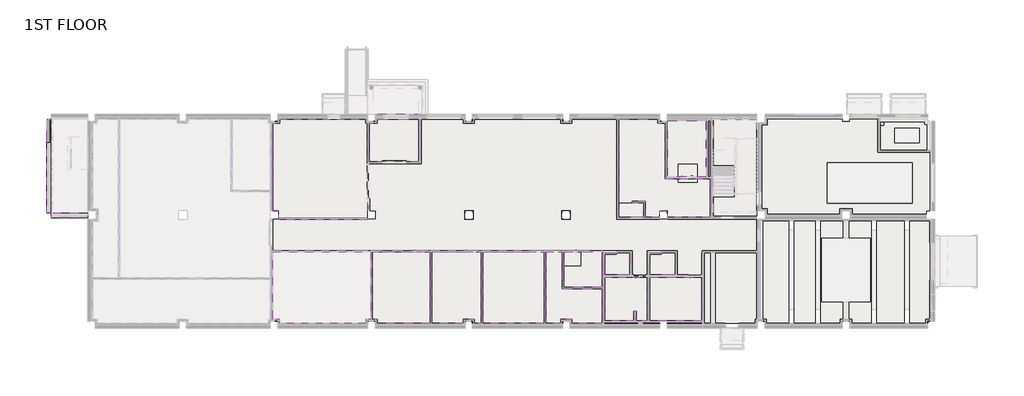
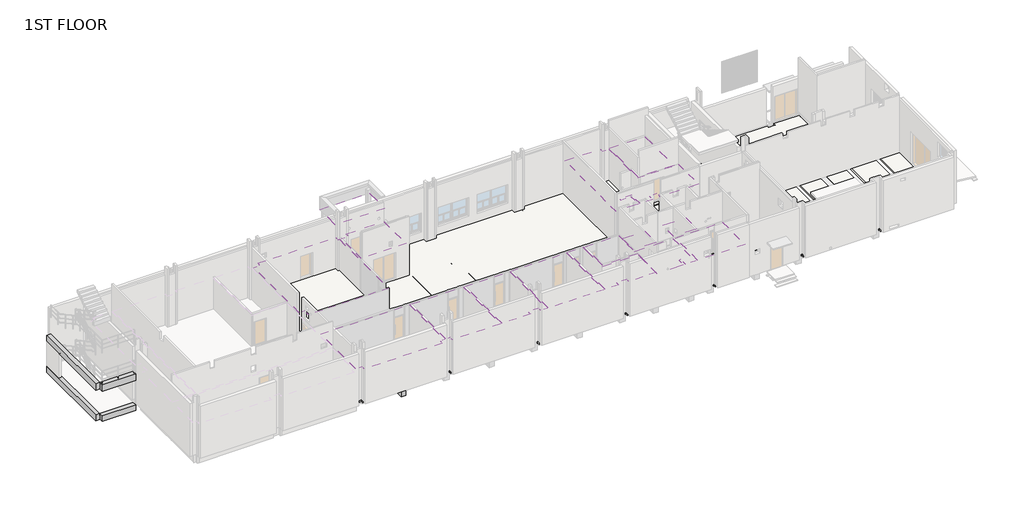
# One storey, part 8 of 15: 26 slabs, 15 coverings, 5 beams.
"""IFC4 building model written with IfcOpenShell, lengths in millimetres."""

from ifc_helpers import new_model, si_unit, frame, origin, place, context, project, spatial, polyline, outline, extrude, faceted_brep, element, save

model = new_model("IFC4")

# Units and contexts
model_context = context("Model", 3, world=origin())
ifc_project = project(units=[si_unit("LENGTHUNIT", "METRE", prefix="MILLI")], contexts=[model_context])

# Site, building, storey
site = spatial("IfcSite", under=ifc_project)
building = spatial("IfcBuilding", under=site)
storey = spatial("IfcBuildingStorey", under=building, Name="1ST FLOOR", Elevation=4800.0)

# Beams
placement = place(None, origin())
element("IfcBeam", 1, ObjectType="RC Beam_Rectangular : H_SB_AR S16_TG-UG_450x800_1B1A", at=placement, inside=storey, context=model_context, shape_type="Brep", body=[
    faceted_brep([(18775.0, -16900.0, 4800.0), (19225.0, -16900.0, 4800.0), (19225.0, -8350.0, 4800.0), (18775.0, -8350.0, 4800.0), (19225.0, -16900.0, 4650.0), (19225.0, -16900.0, 4000.0), (19225.0, -8350.0, 4000.0), (19225.0, -8350.0, 4650.0), (18775.0, -16900.0, 4000.0), (18775.0, -8350.0, 4000.0), (18775.0, -8350.0, 4650.0), (18775.0, -16900.0, 4650.0)], [[[0, 1, 2, 3]], [[2, 1, 4, 5, 6, 7]], [[5, 8, 9, 6]], [[0, 3, 10, 9, 8, 11]], [[1, 0, 11, 8, 5, 4]], [[3, 2, 7, 6, 9, 10]]]),
])
element("IfcBeam", 2, ObjectType="RC Beam_Rectangular : H_SB_AR S16_RC Beam-AG_400x530_SG1A", at=placement, inside=storey, context=model_context, shape_type="Brep", body=[
    faceted_brep([(-300.0, -8200.0, 4630.0), (-300.0, -7800.0, 4630.0), (-3300.0, -7800.0, 4630.0), (-3300.0, -8200.0, 4630.0), (-300.0, -8200.0, 4100.0), (-3300.0, -8200.0, 4100.0), (-300.0, -7800.0, 4100.0), (-3300.0, -7800.0, 4100.0), (-300.0, -7800.0, 4430.0), (-3300.0, -7800.0, 4430.0)], [[[0, 1, 2, 3]], [[4, 0, 3, 5]], [[6, 4, 5, 7]], [[1, 8, 6, 7, 9, 2]], [[1, 0, 4, 6, 8]], [[2, 9, 7, 5, 3]]]),
])
element("IfcBeam", 3, ObjectType="RC Beam_Rectangular : H_SB_AR S16_RC Beam-AG_400x600_SG2", at=placement, inside=storey, context=model_context, shape_type="Brep", body=[
    faceted_brep([(-3700.0, -7800.0, 4630.0), (-3300.0, -7800.0, 4630.0), (-3300.0, -100.0, 4630.0), (-3450.0, -100.0, 4630.0), (-3700.0, -100.0, 4630.0), (-3700.0, -2000.0, 4630.0), (-3700.0, -7800.0, 4030.0), (-3700.0, -100.0, 4030.0), (-3300.0, -7800.0, 4030.0), (-3300.0, -100.0, 4030.0), (-3300.0, -7800.0, 4430.0), (-3300.0, -100.0, 4430.0)], [[[0, 1, 2, 3, 4, 5]], [[6, 0, 5, 4, 7]], [[8, 6, 7, 9]], [[1, 10, 8, 9, 11, 2]], [[1, 0, 6, 8, 10]], [[4, 3, 2, 11, 9, 7]]]),
])
element("IfcBeam", 4, ObjectType="RC Beam_Rectangular : H_SB_AR S16_RC Beam-AG_400x600_SWG2", at=placement, inside=storey, context=model_context, shape_type="Brep", body=[
    faceted_brep([(-3700.0, -7800.0, 7590.0), (-3300.0, -7800.0, 7590.0), (-3300.0, -100.0, 7590.0), (-3450.0, -100.0, 7590.0), (-3700.0, -100.0, 7590.0), (-3700.0, -2000.0, 7590.0), (-3300.0, -7800.0, 6990.0), (-3300.0, -100.0, 6990.0), (-3700.0, -7800.0, 6990.0), (-3700.0, -2000.0, 6990.0), (-3700.0, -100.0, 6990.0), (-3450.0, -100.0, 6990.0)], [[[0, 1, 2, 3, 4, 5]], [[1, 6, 7, 2]], [[6, 8, 9, 10, 11, 7]], [[8, 0, 5, 4, 10, 9]], [[1, 0, 8, 6]], [[4, 3, 2, 7, 11, 10]]]),
])
element("IfcBeam", 5, ObjectType="RC Beam_Rectangular : H_SB_AR S16_RC Beam-AG_400x600_SG1", at=placement, inside=storey, context=model_context, shape_type="SweptSolid", body=[
    extrude(outline(polyline([(-300.0, -7800.0), (-300.0, -8200.0), (-3300.0, -8200.0), (-3300.0, -7800.0), (-300.0, -7800.0)])), frame((0.0, 0.0, 6990.0), z_axis=(0.0, 0.0, 1.0), x_axis=(1.0, 0.0, 0.0)), (0.0, 0.0, 1.0), 600.0),
])

# Coverings
element("IfcCovering", 6, ObjectType="H_CE_AR_B09_2L Gypsum Board_T Bar_9T_C4", at=placement, inside=storey, context=model_context, shape_type="SweptSolid", body=[
    extrude(outline(polyline([(22536.0, -114.0), (22536.0, -464.0), (22649.9999955, -464.0), (22649.9999955, -8250.0), (15400.0000001, -8250.0), (15400.0000001, -7650.0), (14886.0, -7650.0), (14886.0, -464.0), (15464.0, -464.0), (15464.0, -114.0), (22536.0, -114.0)])), frame((0.0, 0.0, 7830.0), z_axis=(0.0, 0.0, 1.0), x_axis=(1.0, 0.0, 0.0)), (0.0, 0.0, 1.0), 19.0),
])
element("IfcCovering", 7, ObjectType="H_CE_AR_B09_Aluminum Spandrel_M Bar_0.8T_C9", at=placement, inside=storey, context=model_context, shape_type="SweptSolid", body=[
    extrude(outline(polyline([(22836.0, -464.0), (23464.0, -464.0), (23464.0, -114.0), (26907.0, -114.0), (26907.0, -3607.0), (22836.0, -3607.0), (22836.0, -464.0)])), frame((0.0, 0.0, 7830.0), z_axis=(0.0, 0.0, 1.0), x_axis=(1.0, 0.0, 0.0)), (0.0, 0.0, 1.0), 0.8),
])
element("IfcCovering", 8, ObjectType="H_CE_AR_B09_2L Gypsum Board_T Bar_9T_C4", at=placement, inside=storey, context=model_context, shape_type="SweptSolid", body=[
    extrude(outline(polyline([(43343.0, -114.0), (46536.0, -114.0), (46536.0, -464.0), (47132.0, -464.0), (47132.0, -4993.0), (50825.0, -4993.0), (50825.0, -8164.0), (47349.9999999, -8164.0), (47349.9999999, -7650.0), (46649.9999999, -7650.0), (46649.9999999, -8164.0), (45514.0, -8164.0), (45514.0, -6836.0), (44443.0, -6836.0), (44443.0, -6964.0), (45386.0, -6964.0), (45386.0, -8164.0), (43343.0, -8164.0), (43343.0, -114.0)])), frame((0.0, 0.0, 7910.0), z_axis=(0.0, 0.0, 1.0), x_axis=(1.0, 0.0, 0.0)), (0.0, 0.0, 1.0), 19.0),
])
element("IfcCovering", 9, ObjectType="H_CE_AR_B09_SMC Ceiling_T Bar_300x300x0.8T_C6", at=placement, inside=storey, context=model_context, shape_type="SweptSolid", body=[
    extrude(outline(polyline([(50525.0, -4825.0), (47300.0, -4825.0), (47300.0, -250.0), (50525.0, -250.0), (50525.0, -4825.0)])), frame((0.0, 0.0, 7800.0), z_axis=(0.0, 0.0, 1.0), x_axis=(1.0, 0.0, 0.0)), (0.0, 0.0, 1.0), 0.8),
])
element("IfcCovering", 10, ObjectType="H_CE_AR_B09_2L Gypsum Board_T Bar_9T_C4", at=placement, inside=storey, context=model_context, shape_type="SweptSolid", body=[
    extrude(outline(polyline([(14886.0, -11007.0000083), (22936.0, -11007.0000083), (22936.0, -16536.0), (22536.0, -16536.0), (22536.0, -16886.0), (15464.0, -16886.0), (15464.0, -16536.0), (14886.0, -16536.0), (14886.0, -11007.0000083)])), frame((0.0, 0.0, 7830.0), z_axis=(0.0, 0.0, 1.0), x_axis=(1.0, 0.0, 0.0)), (0.0, 0.0, 1.0), 19.0),
])
element("IfcCovering", 11, ObjectType="H_CE_AR_B09_2L Gypsum Board_T Bar_9T_C4", at=placement, inside=storey, context=model_context, shape_type="SweptSolid", body=[
    extrude(outline(polyline([(23464.0, -16886.0), (23464.0, -16536.0), (23064.0, -16536.0), (23064.0, -11007.0), (27836.0, -11007.0), (27836.0, -16886.0), (23464.0, -16886.0)])), frame((0.0, 0.0, 7830.0), z_axis=(0.0, 0.0, 1.0), x_axis=(1.0, 0.0, 0.0)), (0.0, 0.0, 1.0), 19.0),
])
element("IfcCovering", 12, ObjectType="H_CE_AR_B09_Souns Absorbing Soft Fiber Board_T Bar_600x600x9T_C5", at=placement, inside=storey, context=model_context, shape_type="SweptSolid", body=[
    extrude(outline(polyline([(27964.0, -11007.0), (32036.0, -11007.0), (32036.0, -16886.0), (31464.0, -16886.0), (31464.0, -16536.0), (30536.0, -16536.0), (30536.0, -16886.0), (27964.0, -16886.0), (27964.0, -11007.0)])), frame((0.0, 0.0, 7830.0), z_axis=(0.0, 0.0, 1.0), x_axis=(1.0, 0.0, 0.0)), (0.0, 0.0, 1.0), 9.0),
])
element("IfcCovering", 13, ObjectType="H_CE_AR_B09_2L Gypsum Board_T Bar_9T_C4", at=placement, inside=storey, context=model_context, shape_type="SweptSolid", body=[
    extrude(outline(polyline([(37186.0, -11007.0), (37186.0, -16886.0), (32164.0, -16886.0), (32164.0, -11007.0), (37186.0, -11007.0)])), frame((0.0, 0.0, 7830.0), z_axis=(0.0, 0.0, 1.0), x_axis=(1.0, 0.0, 0.0)), (0.0, 0.0, 1.0), 19.0),
])
element("IfcCovering", 14, ObjectType="H_CE_AR_B09_Souns Absorbing Soft Fiber Board_T Bar_600x600x9T_C5", at=placement, inside=storey, context=model_context, shape_type="SweptSolid", body=[
    extrude(outline(polyline([(38686.0000001, -14064.0), (41957.0, -14064.0), (41957.0, -16886.0), (39464.0, -16886.0), (39464.0, -16536.0), (38536.0, -16536.0), (38536.0, -16886.0), (37314.0, -16886.0), (37314.0, -11007.0000083), (38686.0000001, -11007.0000083), (38686.0000001, -14064.0)])), frame((0.0, 0.0, 7830.0), z_axis=(0.0, 0.0, 1.0), x_axis=(1.0, 0.0, 0.0)), (0.0, 0.0, 1.0), 9.0),
])
element("IfcCovering", 15, ObjectType="H_CE_AR_B09_Souns Absorbing Soft Fiber Board_T Bar_600x600x9T_C5", at=placement, inside=storey, context=model_context, shape_type="SweptSolid", body=[
    extrude(outline(polyline([(41957.0, -11007.0), (41957.0, -13936.0), (38814.0000001, -13936.0), (38814.0000001, -11007.0), (41957.0, -11007.0)])), frame((0.0, 0.0, 7830.0), z_axis=(0.0, 0.0, 1.0), x_axis=(1.0, 0.0, 0.0)), (0.0, 0.0, 1.0), 9.0),
])
element("IfcCovering", 16, ObjectType="H_CE_AR_B09_2L Gypsum Board_T Bar_9T_C4", at=placement, inside=storey, context=model_context, shape_type="SweptSolid", body=[
    extrude(outline(polyline([(44245.0, -12895.0), (42155.0, -12895.0), (42155.0, -11105.0), (44245.0, -11105.0), (44245.0, -12895.0)])), frame((0.0, 0.0, 7500.0), z_axis=(0.0, 0.0, 1.0), x_axis=(1.0, 0.0, 0.0)), (0.0, 0.0, 1.0), 19.0),
])
element("IfcCovering", 17, ObjectType="H_CE_AR_B09_2L Gypsum Board_T Bar_9T_C4", at=placement, inside=storey, context=model_context, shape_type="SweptSolid", body=[
    extrude(outline(polyline([(45645.0, -13105.0), (45645.0, -16670.0), (44755.0, -16670.0), (44755.0, -15905.0), (44545.0, -15905.0), (44545.0, -16670.0), (42155.0, -16670.0), (42155.0, -13105.0), (45645.0, -13105.0)])), frame((0.0, 0.0, 7500.0), z_axis=(0.0, 0.0, 1.0), x_axis=(1.0, 0.0, 0.0)), (0.0, 0.0, 1.0), 19.0),
])
element("IfcCovering", 18, ObjectType="H_CE_AR_B09_2L Gypsum Board_T Bar_9T_C4", at=placement, inside=storey, context=model_context, shape_type="SweptSolid", body=[
    extrude(outline(polyline([(50145.0, -13105.0), (50145.0, -16670.0), (45855.0, -16670.0), (45855.0, -13105.0), (50145.0, -13105.0)])), frame((0.0, 0.0, 7500.0), z_axis=(0.0, 0.0, 1.0), x_axis=(1.0, 0.0, 0.0)), (0.0, 0.0, 1.0), 19.0),
])
element("IfcCovering", 19, ObjectType="H_CE_AR_B09_2L Gypsum Board_T Bar_9T_C4", at=placement, inside=storey, context=model_context, shape_type="SweptSolid", body=[
    extrude(outline(polyline([(47945.0, -11105.0000016), (47945.0, -12895.0), (45855.0, -12895.0), (45855.0, -11105.0000016), (47945.0, -11105.0000016)])), frame((0.0, 0.0, 7500.0), z_axis=(0.0, 0.0, 1.0), x_axis=(1.0, 0.0, 0.0)), (0.0, 0.0, 1.0), 19.0),
])
element("IfcCovering", 20, ObjectType="H_CE_AR_B09_Stainless Hairline Finish_3T", at=placement, inside=storey, context=model_context, shape_type="SweptSolid", body=[
    extrude(outline(polyline([(27247.0, 2747.0), (27247.0, 300.0), (22753.0, 300.0), (22753.0, 2747.0), (27247.0, 2747.0)]), holes=[polyline([(23150.0, 2650.0), (22850.0, 2650.0), (22850.0, 2350.0), (23150.0, 2350.0), (23150.0, 2650.0)]), polyline([(26850.0, 2650.0), (26850.0, 2350.0), (27150.0, 2350.0), (27150.0, 2650.0), (26850.0, 2650.0)])]), frame((0.0, 0.0, 8700.0), z_axis=(0.0, 0.0, 1.0), x_axis=(1.0, 0.0, 0.0)), (0.0, 0.0, 1.0), 3.0),
])

# Slabs
element("IfcSlab", 21, ObjectType="H_FL_AR_S17_RC Slab_T150_1S1", at=placement, inside=storey, context=model_context, shape_type="Brep", body=[
    faceted_brep([(18775.0, -100.0, 4650.0), (18775.0, -7850.0, 4650.0), (15400.0000001, -7850.0, 4650.0), (15400.0000001, -7650.0, 4650.0), (15100.0, -7650.0, 4650.0), (15100.0, -300.0, 4650.0), (15300.0, -300.0, 4650.0), (15300.0, -100.0, 4650.0), (18775.0, -7850.0, 4800.0), (18775.0, -100.0, 4800.0), (15300.0, -100.0, 4800.0), (15300.0, -300.0, 4800.0), (15100.0, -300.0, 4800.0), (15100.0, -7650.0, 4800.0), (15400.0000001, -7650.0, 4800.0), (15400.0000001, -7850.0, 4800.0)], [[[0, 1, 2, 3, 4, 5, 6, 7]], [[8, 9, 10, 11, 12, 13, 14, 15]], [[1, 0, 9, 8]], [[2, 1, 8, 15]], [[3, 2, 15, 14]], [[4, 3, 14, 13]], [[5, 4, 13, 12]], [[0, 7, 10, 9]], [[6, 5, 12, 11]], [[7, 6, 11, 10]]]),
    faceted_brep([(18775.0, -16900.0, 4650.0), (15300.0, -16900.0, 4650.0), (15300.0, -16700.0, 4650.0), (15100.0, -16700.0, 4650.0), (15100.0, -8350.0, 4650.0), (18775.0, -8350.0, 4650.0), (15300.0, -16900.0, 4800.0), (18775.0, -16900.0, 4800.0), (18775.0, -8350.0, 4800.0), (15400.0000001, -8350.0, 4800.0), (15100.0, -8350.0, 4800.0), (15100.0, -16700.0, 4800.0), (15300.0, -16700.0, 4800.0)], [[[0, 1, 2, 3, 4, 5]], [[6, 7, 8, 9, 10, 11, 12]], [[1, 0, 7, 6]], [[2, 1, 6, 12]], [[3, 2, 12, 11]], [[4, 3, 11, 10]], [[5, 4, 10, 9, 8]], [[0, 5, 8, 7]]]),
    faceted_brep([(22650.0000003, -7850.0, 4650.0), (19225.0, -7850.0, 4650.0), (19225.0, -100.0, 4650.0), (22700.0, -100.0, 4650.0), (22700.0, -7650.0, 4650.0), (22650.0000003, -7650.0, 4650.0), (19225.0, -7850.0, 4800.0), (22650.0000003, -7850.0, 4800.0), (22650.0000003, -7650.0, 4800.0), (22700.0, -7650.0, 4800.0), (22700.0, -300.0, 4800.0), (22700.0, -100.0, 4800.0), (19225.0, -100.0, 4800.0)], [[[0, 1, 2, 3, 4, 5]], [[6, 7, 8, 9, 10, 11, 12]], [[1, 0, 7, 6]], [[2, 1, 6, 12]], [[3, 2, 12, 11]], [[4, 3, 11, 10, 9]], [[5, 4, 9, 8]], [[0, 5, 8, 7]]]),
    faceted_brep([(19225.0, -8350.0, 4650.0), (22750.0, -8350.0, 4650.0), (22750.0, -16700.0, 4650.0), (22700.0, -16700.0, 4650.0), (22700.0, -16900.0, 4650.0), (19225.0, -16900.0, 4650.0), (22750.0, -8350.0, 4800.0), (22650.0, -8350.0, 4800.0), (19225.0, -8350.0, 4800.0), (19225.0, -16900.0, 4800.0), (22700.0, -16900.0, 4800.0), (22700.0, -16700.0, 4800.0), (22750.0, -16700.0, 4800.0)], [[[0, 1, 2, 3, 4, 5]], [[6, 7, 8, 9, 10, 11, 12]], [[1, 0, 8, 7, 6]], [[2, 1, 6, 12]], [[3, 2, 12, 11]], [[4, 3, 11, 10]], [[5, 4, 10, 9]], [[0, 5, 9, 8]]]),
    faceted_brep([(26775.0, -8350.0, 4650.0), (26775.0, -16900.0, 4650.0), (23300.0, -16900.0, 4650.0), (23300.0, -16700.0, 4650.0), (23250.0, -16700.0, 4650.0), (23250.0, -8350.0, 4650.0), (26775.0, -16900.0, 4800.0), (26775.0, -8350.0, 4800.0), (23350.0, -8350.0, 4800.0), (23250.0, -8350.0, 4800.0), (23250.0, -16700.0, 4800.0), (23300.0, -16700.0, 4800.0), (23300.0, -16900.0, 4800.0)], [[[0, 1, 2, 3, 4, 5]], [[6, 7, 8, 9, 10, 11, 12]], [[1, 0, 7, 6]], [[2, 1, 6, 12]], [[3, 2, 12, 11]], [[4, 3, 11, 10]], [[5, 4, 10, 9]], [[0, 5, 9, 8, 7]]]),
    faceted_brep([(23350.0000003, -7850.0, 4650.0), (23350.0000003, -7650.0, 4650.0), (23200.0, -7650.0, 4650.0), (23200.0, -300.0, 4650.0), (23300.0, -300.0, 4650.0), (23300.0, -100.0, 4650.0), (26775.0, -100.0, 4650.0), (26775.0, -7850.0, 4650.0), (23350.0000003, -7650.0, 4800.0), (23350.0000003, -7850.0, 4800.0), (26775.0, -7850.0, 4800.0), (26775.0, -100.0, 4800.0), (23300.0, -100.0, 4800.0), (23300.0, -300.0, 4800.0), (23200.0, -300.0, 4800.0), (23200.0, -7650.0, 4800.0)], [[[0, 1, 2, 3, 4, 5, 6, 7]], [[8, 9, 10, 11, 12, 13, 14, 15]], [[1, 0, 9, 8]], [[2, 1, 8, 15]], [[3, 2, 15, 14]], [[4, 3, 14, 13]], [[5, 4, 13, 12]], [[6, 5, 12, 11]], [[7, 6, 11, 10]], [[0, 7, 10, 9]]]),
    faceted_brep([(30700.0, -100.0, 4650.0), (30700.0, -300.0, 4650.0), (30750.0, -300.0, 4650.0), (30750.0, -7650.0, 4650.0), (30650.0000002, -7650.0, 4650.0), (30650.0000002, -7850.0, 4650.0), (27225.0, -7850.0, 4650.0), (27225.0, -100.0, 4650.0), (30700.0, -300.0, 4800.0), (30700.0, -100.0, 4800.0), (27225.0, -100.0, 4800.0), (27225.0, -7850.0, 4800.0), (30650.0000002, -7850.0, 4800.0), (30650.0000002, -7650.0, 4800.0), (30750.0, -7650.0, 4800.0), (30750.0, -300.0, 4800.0)], [[[0, 1, 2, 3, 4, 5, 6, 7]], [[8, 9, 10, 11, 12, 13, 14, 15]], [[1, 0, 9, 8]], [[2, 1, 8, 15]], [[3, 2, 15, 14]], [[4, 3, 14, 13]], [[5, 4, 13, 12]], [[6, 5, 12, 11]], [[7, 6, 11, 10]], [[0, 7, 10, 9]]]),
    faceted_brep([(30700.0, -16900.0, 4650.0), (27225.0, -16900.0, 4650.0), (27225.0, -8350.0, 4650.0), (30750.0, -8350.0, 4650.0), (30750.0, -16700.0, 4650.0), (30700.0, -16700.0, 4650.0), (27225.0, -16900.0, 4800.0), (30700.0, -16900.0, 4800.0), (30700.0, -16700.0, 4800.0), (30750.0, -16700.0, 4800.0), (30750.0, -8350.0, 4800.0), (30650.0, -8350.0, 4800.0), (27225.0, -8350.0, 4800.0)], [[[0, 1, 2, 3, 4, 5]], [[6, 7, 8, 9, 10, 11, 12]], [[1, 0, 7, 6]], [[2, 1, 6, 12]], [[3, 2, 12, 11, 10]], [[4, 3, 10, 9]], [[5, 4, 9, 8]], [[0, 5, 8, 7]]]),
    faceted_brep([(31300.0, -16900.0, 4650.0), (31300.0, -16700.0, 4650.0), (31250.0, -16700.0, 4650.0), (31250.0, -8350.0, 4650.0), (34775.0, -8350.0, 4650.0), (34775.0, -16900.0, 4650.0), (31300.0, -16700.0, 4800.0), (31300.0, -16900.0, 4800.0), (34775.0, -16900.0, 4800.0), (34775.0, -8350.0, 4800.0), (31350.0, -8350.0, 4800.0), (31250.0, -8350.0, 4800.0), (31250.0, -16700.0, 4800.0)], [[[0, 1, 2, 3, 4, 5]], [[6, 7, 8, 9, 10, 11, 12]], [[1, 0, 7, 6]], [[2, 1, 6, 12]], [[3, 2, 12, 11]], [[4, 3, 11, 10, 9]], [[5, 4, 9, 8]], [[0, 5, 8, 7]]]),
    faceted_brep([(31300.0, -100.0, 4650.0), (34775.0, -100.0, 4650.0), (34775.0, -7850.0, 4650.0), (31349.9999998, -7850.0, 4650.0), (31349.9999998, -7650.0, 4650.0), (31250.0, -7650.0, 4650.0), (31250.0, -300.0, 4650.0), (31300.0, -300.0, 4650.0), (34775.0, -100.0, 4800.0), (31300.0, -100.0, 4800.0), (31300.0, -300.0, 4800.0), (31250.0, -300.0, 4800.0), (31250.0, -7650.0, 4800.0), (31349.9999998, -7650.0, 4800.0), (31349.9999998, -7850.0, 4800.0), (34775.0, -7850.0, 4800.0)], [[[0, 1, 2, 3, 4, 5, 6, 7]], [[8, 9, 10, 11, 12, 13, 14, 15]], [[1, 0, 9, 8]], [[2, 1, 8, 15]], [[3, 2, 15, 14]], [[4, 3, 14, 13]], [[5, 4, 13, 12]], [[6, 5, 12, 11]], [[7, 6, 11, 10]], [[0, 7, 10, 9]]]),
    faceted_brep([(38700.0, -16900.0, 4650.0), (35225.0, -16900.0, 4650.0), (35225.0, -8350.0, 4650.0), (38750.0, -8350.0, 4650.0), (38750.0, -16700.0, 4650.0), (38700.0, -16700.0, 4650.0), (35225.0, -16900.0, 4800.0), (38700.0, -16900.0, 4800.0), (38700.0, -16700.0, 4800.0), (38750.0, -16700.0, 4800.0), (38750.0, -8350.0, 4800.0), (38650.0, -8350.0, 4800.0), (35225.0, -8350.0, 4800.0)], [[[0, 1, 2, 3, 4, 5]], [[6, 7, 8, 9, 10, 11, 12]], [[1, 0, 7, 6]], [[2, 1, 6, 12]], [[3, 2, 12, 11, 10]], [[4, 3, 10, 9]], [[5, 4, 9, 8]], [[0, 5, 8, 7]]]),
    faceted_brep([(38700.0, -100.0, 4650.0), (38700.0, -300.0, 4650.0), (38750.0, -300.0, 4650.0), (38750.0, -7650.0, 4650.0), (38650.0000002, -7650.0, 4650.0), (38650.0000002, -7850.0, 4650.0), (35225.0, -7850.0, 4650.0), (35225.0, -100.0, 4650.0), (38700.0, -300.0, 4800.0), (38700.0, -100.0, 4800.0), (35225.0, -100.0, 4800.0), (35225.0, -7850.0, 4800.0), (38650.0000002, -7850.0, 4800.0), (38650.0000002, -7650.0, 4800.0), (38750.0, -7650.0, 4800.0), (38750.0, -300.0, 4800.0)], [[[0, 1, 2, 3, 4, 5, 6, 7]], [[8, 9, 10, 11, 12, 13, 14, 15]], [[1, 0, 9, 8]], [[2, 1, 8, 15]], [[3, 2, 15, 14]], [[4, 3, 14, 13]], [[5, 4, 13, 12]], [[6, 5, 12, 11]], [[7, 6, 11, 10]], [[0, 7, 10, 9]]]),
    faceted_brep([(39300.0, -16900.0, 4650.0), (39300.0, -16700.0, 4650.0), (39250.0, -16700.0, 4650.0), (39250.0, -8350.0, 4650.0), (41675.0, -8350.0, 4650.0), (41675.0, -16900.0, 4650.0), (39300.0, -16700.0, 4800.0), (39300.0, -16900.0, 4800.0), (41675.0, -16900.0, 4800.0), (41675.0, -8350.0, 4800.0), (39350.0, -8350.0, 4800.0), (39250.0, -8350.0, 4800.0), (39250.0, -16700.0, 4800.0)], [[[0, 1, 2, 3, 4, 5]], [[6, 7, 8, 9, 10, 11, 12]], [[1, 0, 7, 6]], [[2, 1, 6, 12]], [[3, 2, 12, 11]], [[4, 3, 11, 10, 9]], [[5, 4, 9, 8]], [[0, 5, 8, 7]]]),
    faceted_brep([(39300.0, -100.0, 4650.0), (41675.0, -100.0, 4650.0), (41675.0, -7850.0, 4650.0), (39349.9999998, -7850.0, 4650.0), (39349.9999998, -7650.0, 4650.0), (39250.0, -7650.0, 4650.0), (39250.0, -300.0, 4650.0), (39300.0, -300.0, 4650.0), (41675.0, -100.0, 4800.0), (39300.0, -100.0, 4800.0), (39300.0, -300.0, 4800.0), (39250.0, -300.0, 4800.0), (39250.0, -7650.0, 4800.0), (39349.9999998, -7650.0, 4800.0), (39349.9999998, -7850.0, 4800.0), (41675.0, -7850.0, 4800.0)], [[[0, 1, 2, 3, 4, 5, 6, 7]], [[8, 9, 10, 11, 12, 13, 14, 15]], [[1, 0, 9, 8]], [[2, 1, 8, 15]], [[3, 2, 15, 14]], [[4, 3, 14, 13]], [[5, 4, 13, 12]], [[6, 5, 12, 11]], [[7, 6, 11, 10]], [[0, 7, 10, 9]]]),
    faceted_brep([(42125.0, -100.0, 4650.0), (44875.0, -100.0, 4650.0), (44875.0, -7850.0, 4650.0), (42125.0, -7850.0, 4650.0), (44875.0, -100.0, 4800.0), (42125.0, -100.0, 4800.0), (42125.0, -7850.0, 4800.0), (44875.0, -7850.0, 4800.0)], [[[0, 1, 2, 3]], [[4, 5, 6, 7]], [[1, 0, 5, 4]], [[2, 1, 4, 7]], [[3, 2, 7, 6]], [[0, 3, 6, 5]]]),
    faceted_brep([(46649.9999999, -7850.0, 4650.0), (45325.0, -7850.0, 4650.0), (45325.0, -100.0, 4650.0), (46700.0, -100.0, 4650.0), (46700.0, -300.0, 4650.0), (46800.0, -300.0, 4650.0), (46800.0, -7650.0, 4650.0), (46649.9999999, -7650.0, 4650.0), (45325.0, -7850.0, 4800.0), (46649.9999999, -7850.0, 4800.0), (46649.9999999, -7650.0, 4800.0), (46800.0, -7650.0, 4800.0), (46800.0, -300.0, 4800.0), (46700.0, -300.0, 4800.0), (46700.0, -100.0, 4800.0), (45325.0, -100.0, 4800.0)], [[[0, 1, 2, 3, 4, 5, 6, 7]], [[8, 9, 10, 11, 12, 13, 14, 15]], [[1, 0, 9, 8]], [[2, 1, 8, 15]], [[3, 2, 15, 14]], [[4, 3, 14, 13]], [[5, 4, 13, 12]], [[6, 5, 12, 11]], [[7, 6, 11, 10]], [[0, 7, 10, 9]]]),
    faceted_brep([(50825.0, -4825.0, 4650.0), (50825.0, -7850.0, 4650.0), (47349.9999999, -7850.0, 4650.0), (47300.0, -7850.0, 4650.0), (47300.0, -7650.0, 4650.0), (47300.0, -4825.0, 4650.0), (50825.0, -7850.0, 4800.0), (50825.0, -4825.0, 4800.0), (47300.0, -4825.0, 4800.0), (47300.0, -7650.0, 4800.0), (47300.0, -7850.0, 4800.0), (47349.9999999, -7850.0, 4800.0), (50825.0, -4825.0, 4700.0), (47300.0, -4825.0, 4700.0)], [[[0, 1, 2, 3, 4, 5]], [[6, 7, 8, 9, 10, 11]], [[1, 0, 12, 7, 6]], [[3, 2, 1, 6, 11, 10]], [[5, 4, 3, 10, 9, 8, 13]], [[0, 5, 13, 8, 7, 12]]]),
    faceted_brep([(54700.0, -8350.0, 4650.0), (54700.0, -16900.0, 4650.0), (51275.0, -16900.0, 4650.0), (51275.0, -8350.0, 4650.0), (54700.0, -16900.0, 4800.0), (54700.0, -16700.0, 4800.0), (54700.0, -8350.0, 4800.0), (51275.0, -8350.0, 4800.0), (51275.0, -16900.0, 4800.0)], [[[0, 1, 2, 3]], [[4, 5, 6, 7, 8]], [[1, 0, 6, 5, 4]], [[2, 1, 4, 8]], [[3, 2, 8, 7]], [[0, 3, 7, 6]]]),
    faceted_brep([(57275.0, -8350.0, 4650.0), (57275.0, -16900.0, 4650.0), (55300.0, -16900.0, 4650.0), (55300.0, -16700.0, 4650.0), (55200.0, -16700.0, 4650.0), (55200.0, -8350.0, 4650.0), (57275.0, -16900.0, 4800.0), (57275.0, -8350.0, 4800.0), (55200.0, -8350.0, 4800.0), (55200.0, -16700.0, 4800.0), (55300.0, -16700.0, 4800.0), (55300.0, -16900.0, 4800.0)], [[[0, 1, 2, 3, 4, 5]], [[6, 7, 8, 9, 10, 11]], [[1, 0, 7, 6]], [[2, 1, 6, 11]], [[3, 2, 11, 10]], [[4, 3, 10, 9]], [[5, 4, 9, 8]], [[0, 5, 8, 7]]]),
    faceted_brep([(59475.0, -8350.0, 4650.0), (59475.0, -16900.0, 4650.0), (57725.0, -16900.0, 4650.0), (57725.0, -8350.0, 4650.0), (59475.0, -16900.0, 4800.0), (59475.0, -8350.0, 4800.0), (57725.0, -8350.0, 4800.0), (57725.0, -16900.0, 4800.0)], [[[0, 1, 2, 3]], [[4, 5, 6, 7]], [[1, 0, 5, 4]], [[2, 1, 4, 7]], [[3, 2, 7, 6]], [[0, 3, 6, 5]]]),
    faceted_brep([(61750.0, -8350.0, 4650.0), (61750.0, -16700.0, 4650.0), (61700.0, -16700.0, 4650.0), (61700.0, -16900.0, 4650.0), (59925.0, -16900.0, 4650.0), (59925.0, -8350.0, 4650.0), (61750.0, -16700.0, 4800.0), (61750.0, -8350.0, 4800.0), (59925.0, -8350.0, 4800.0), (59925.0, -16900.0, 4800.0), (61700.0, -16900.0, 4800.0), (61700.0, -16700.0, 4800.0)], [[[0, 1, 2, 3, 4, 5]], [[6, 7, 8, 9, 10, 11]], [[1, 0, 7, 6]], [[2, 1, 6, 11]], [[3, 2, 11, 10]], [[4, 3, 10, 9]], [[5, 4, 9, 8]], [[0, 5, 8, 7]]]),
    faceted_brep([(62250.0, -8350.0, 4650.0), (64075.0, -8350.0, 4650.0), (64075.0, -16900.0, 4650.0), (62300.0, -16900.0, 4650.0), (62300.0, -16700.0, 4650.0), (62250.0, -16700.0, 4650.0), (64075.0, -8350.0, 4800.0), (62250.0, -8350.0, 4800.0), (62250.0, -16700.0, 4800.0), (62300.0, -16700.0, 4800.0), (62300.0, -16900.0, 4800.0), (64075.0, -16900.0, 4800.0)], [[[0, 1, 2, 3, 4, 5]], [[6, 7, 8, 9, 10, 11]], [[1, 0, 7, 6]], [[2, 1, 6, 11]], [[3, 2, 11, 10]], [[4, 3, 10, 9]], [[5, 4, 9, 8]], [[0, 5, 8, 7]]]),
    faceted_brep([(66775.0, -8350.0, 4650.0), (66775.0, -16900.0, 4650.0), (64525.0, -16900.0, 4650.0), (64525.0, -8350.0, 4650.0), (66775.0, -16900.0, 4800.0), (66775.0, -8350.0, 4800.0), (64525.0, -8350.0, 4800.0), (64525.0, -16900.0, 4800.0)], [[[0, 1, 2, 3]], [[4, 5, 6, 7]], [[1, 0, 5, 4]], [[2, 1, 4, 7]], [[3, 2, 7, 6]], [[0, 3, 6, 5]]]),
    faceted_brep([(68700.0, -16900.0, 4650.0), (67225.0, -16900.0, 4650.0), (67225.0, -8350.0, 4650.0), (68900.0, -8350.0, 4650.0), (68900.0, -16700.0, 4650.0), (68700.0, -16700.0, 4650.0), (67225.0, -16900.0, 4800.0), (68700.0, -16900.0, 4800.0), (68700.0, -16700.0, 4800.0), (68900.0, -16700.0, 4800.0), (68900.0, -8350.0, 4800.0), (67225.0, -8350.0, 4800.0)], [[[0, 1, 2, 3, 4, 5]], [[6, 7, 8, 9, 10, 11]], [[1, 0, 7, 6]], [[2, 1, 6, 11]], [[3, 2, 11, 10]], [[4, 3, 10, 9]], [[5, 4, 9, 8]], [[0, 5, 8, 7]]]),
    faceted_brep([(47250.0, -11075.0, 4650.0), (47250.0, -10675.0, 4650.0), (47250.0, -8350.0, 4650.0), (50825.0, -8350.0, 4650.0), (50825.0, -16900.0, 4650.0), (50575.0, -16900.0, 4650.0), (50175.0, -16900.0, 4650.0), (50175.0, -13075.0, 4650.0), (47975.0, -13075.0, 4650.0), (47975.0, -11075.0, 4650.0), (47250.0, -8350.0, 4800.0), (47250.0, -11075.0, 4800.0), (47975.0, -11075.0, 4800.0), (47975.0, -13075.0, 4800.0), (50175.0, -13075.0, 4800.0), (50175.0, -16900.0, 4800.0), (50825.0, -16900.0, 4800.0), (50825.0, -8350.0, 4800.0), (47350.0, -8350.0, 4800.0), (47250.0, -11075.0, 4700.0), (50175.0, -16900.0, 4700.0), (50175.0, -13075.0, 4700.0), (47975.0, -13075.0, 4700.0), (47975.0, -11075.0, 4700.0)], [[[0, 1, 2, 3, 4, 5, 6, 7, 8, 9]], [[10, 11, 12, 13, 14, 15, 16, 17, 18]], [[2, 1, 0, 19, 11, 10]], [[3, 2, 10, 18, 17]], [[4, 3, 17, 16]], [[6, 5, 4, 16, 15, 20]], [[7, 6, 20, 15, 14, 21]], [[8, 7, 21, 14, 13, 22]], [[9, 8, 22, 13, 12, 23]], [[0, 9, 23, 12, 11, 19]]]),
    faceted_brep([(46750.0, -8350.0, 4650.0), (46750.0, -10675.0, 4650.0), (46750.0, -11075.0, 4650.0), (45825.0, -11075.0, 4650.0), (45825.0, -13075.0, 4650.0), (45325.0, -13075.0, 4650.0), (45325.0, -12675.0, 4650.0), (45325.0, -8350.0, 4650.0), (46750.0, -11075.0, 4800.0), (46750.0, -8350.0, 4800.0), (46650.0, -8350.0, 4800.0), (45325.0, -8350.0, 4800.0), (45325.0, -13075.0, 4800.0), (45825.0, -13075.0, 4800.0), (45825.0, -11075.0, 4800.0), (46750.0, -11075.0, 4700.0), (45825.0, -11075.0, 4700.0), (45825.0, -13075.0, 4700.0), (45325.0, -13075.0, 4700.0)], [[[0, 1, 2, 3, 4, 5, 6, 7]], [[8, 9, 10, 11, 12, 13, 14]], [[2, 1, 0, 9, 8, 15]], [[3, 2, 15, 8, 14, 16]], [[4, 3, 16, 14, 13, 17]], [[5, 4, 17, 13, 12, 18]], [[7, 6, 5, 18, 12, 11]], [[0, 7, 11, 10, 9]]]),
    faceted_brep([(44875.0, -8350.0, 4650.0), (44875.0, -12675.0, 4650.0), (44875.0, -13075.0, 4650.0), (44275.0, -13075.0, 4650.0), (44275.0, -11075.0, 4650.0), (42125.0, -11075.0, 4650.0), (42125.0, -10675.0, 4650.0), (42125.0, -8350.0, 4650.0), (44875.0, -13075.0, 4800.0), (44875.0, -8350.0, 4800.0), (42125.0, -8350.0, 4800.0), (42125.0, -11075.0, 4800.0), (44275.0, -11075.0, 4800.0), (44275.0, -13075.0, 4800.0), (44875.0, -13075.0, 4700.0), (44275.0, -13075.0, 4700.0), (44275.0, -11075.0, 4700.0), (42125.0, -11075.0, 4700.0)], [[[0, 1, 2, 3, 4, 5, 6, 7]], [[8, 9, 10, 11, 12, 13]], [[2, 1, 0, 9, 8, 14]], [[3, 2, 14, 8, 13, 15]], [[4, 3, 15, 13, 12, 16]], [[5, 4, 16, 12, 11, 17]], [[7, 6, 5, 17, 11, 10]], [[0, 7, 10, 9]]]),
])
element("IfcSlab", 22, ObjectType="H_FL_AR_S17_RC Slab_T150_1S1", at=placement, inside=storey, context=model_context, shape_type="Brep", body=[
    faceted_brep([(50825.0, -100.0, 4550.0), (50825.0, -4825.0, 4550.0), (47300.0, -4825.0, 4550.0), (47300.0, -100.0, 4550.0), (50825.0, -100.0, 4700.0), (47300.0, -100.0, 4700.0), (47300.0, -4825.0, 4700.0), (50825.0, -4825.0, 4700.0), (50825.0, -4825.0, 4650.0), (47300.0, -4825.0, 4650.0)], [[[0, 1, 2, 3]], [[4, 5, 6, 7]], [[1, 0, 4, 7, 8]], [[2, 1, 8, 7, 6, 9]], [[3, 2, 9, 6, 5]], [[0, 3, 5, 4]]]),
])
element("IfcSlab", 23, ObjectType="H_FL_AR_S17_RC Slab_T150_GS1", at=placement, inside=storey, context=model_context, shape_type="Brep", body=[
    faceted_brep([(62312.0, -112.0, 4650.0), (64707.0, -112.0, 4650.0), (64707.0, -1062.0, 4650.0), (64707.0, -2743.0, 4650.0), (68888.0, -2743.0, 4650.0), (68888.0, -3093.0, 4650.0), (68888.0, -7638.0, 4650.0), (68588.0, -7638.0, 4650.0), (68588.0, -7938.0, 4650.0), (62362.0, -7938.0, 4650.0), (62362.0, -7638.0, 4650.0), (61638.0, -7638.0, 4650.0), (61638.0, -7938.0, 4650.0), (55362.0, -7938.0, 4650.0), (55362.0, -7638.0, 4650.0), (55062.0, -7638.0, 4650.0), (55062.0, -412.0, 4650.0), (55362.0, -412.0, 4650.0), (55362.0, -112.0, 4650.0), (61688.0, -112.0, 4650.0), (61688.0, -312.0, 4650.0), (62312.0, -312.0, 4650.0), (67450.0, -3700.0, 4650.0), (60450.0, -3700.0, 4650.0), (60450.0, -7000.0, 4650.0), (67450.0, -7000.0, 4650.0), (64707.0, -112.0, 4800.0), (62312.0, -112.0, 4800.0), (62312.0, -312.0, 4800.0), (61688.0, -312.0, 4800.0), (61688.0, -112.0, 4800.0), (55362.0, -112.0, 4800.0), (55362.0, -412.0, 4800.0), (55062.0, -412.0, 4800.0), (55062.0, -7638.0, 4800.0), (55362.0, -7638.0, 4800.0), (55362.0, -7938.0, 4800.0), (61638.0, -7938.0, 4800.0), (61638.0, -7638.0, 4800.0), (62362.0, -7638.0, 4800.0), (62362.0, -7938.0, 4800.0), (68588.0, -7938.0, 4800.0), (68588.0, -7638.0, 4800.0), (68888.0, -7638.0, 4800.0), (68888.0, -2743.0, 4800.0), (64707.0, -2743.0, 4800.0), (60450.0, -3700.0, 4800.0), (67450.0, -3700.0, 4800.0), (67450.0, -7000.0, 4800.0), (60450.0, -7000.0, 4800.0)], [[[0, 1, 2, 3, 4, 5, 6, 7, 8, 9, 10, 11, 12, 13, 14, 15, 16, 17, 18, 19, 20, 21], [22, 23, 24, 25]], [[26, 27, 28, 29, 30, 31, 32, 33, 34, 35, 36, 37, 38, 39, 40, 41, 42, 43, 44, 45], [46, 47, 48, 49]], [[1, 0, 27, 26]], [[6, 5, 4, 44, 43]], [[7, 6, 43, 42]], [[8, 7, 42, 41]], [[9, 8, 41, 40]], [[10, 9, 40, 39]], [[11, 10, 39, 38]], [[12, 11, 38, 37]], [[13, 12, 37, 36]], [[14, 13, 36, 35]], [[15, 14, 35, 34]], [[16, 15, 34, 33]], [[17, 16, 33, 32]], [[18, 17, 32, 31]], [[19, 18, 31, 30]], [[20, 19, 30, 29]], [[21, 20, 29, 28]], [[0, 21, 28, 27]], [[23, 22, 47, 46]], [[24, 23, 46, 49]], [[25, 24, 49, 48]], [[22, 25, 48, 47]], [[3, 2, 1, 26, 45]], [[4, 3, 45, 44]]]),
])
element("IfcSlab", 24, ObjectType="H_FL_AR_S17_RC Slab_T150_1S1", at=placement, inside=storey, context=model_context, shape_type="Brep", body=[
    faceted_brep([(47975.0, -11075.0, 4550.0), (47975.0, -13075.0, 4550.0), (50175.0, -13075.0, 4550.0), (50175.0, -16900.0, 4550.0), (47300.0, -16900.0, 4550.0), (47300.0, -16700.0, 4550.0), (47250.0, -16700.0, 4550.0), (47250.0, -11075.0, 4550.0), (47975.0, -11075.0, 4700.0), (47250.0, -11075.0, 4700.0), (47250.0, -16700.0, 4700.0), (47300.0, -16700.0, 4700.0), (47300.0, -16900.0, 4700.0), (50175.0, -16900.0, 4700.0), (50175.0, -13075.0, 4700.0), (47975.0, -13075.0, 4700.0), (47975.0, -11075.0, 4650.0), (47975.0, -13075.0, 4650.0), (50175.0, -13075.0, 4650.0), (50175.0, -16900.0, 4650.0), (47250.0, -11075.0, 4650.0)], [[[0, 1, 2, 3, 4, 5, 6, 7]], [[8, 9, 10, 11, 12, 13, 14, 15]], [[1, 0, 16, 8, 15, 17]], [[2, 1, 17, 15, 14, 18]], [[3, 2, 18, 14, 13, 19]], [[4, 3, 19, 13, 12]], [[5, 4, 12, 11]], [[6, 5, 11, 10]], [[7, 6, 10, 9, 20]], [[0, 7, 20, 9, 8, 16]]]),
    faceted_brep([(45325.0, -13075.0, 4550.0), (45825.0, -13075.0, 4550.0), (45825.0, -11075.0, 4550.0), (46750.0, -11075.0, 4550.0), (46750.0, -16700.0, 4550.0), (46700.0, -16700.0, 4550.0), (46700.0, -16900.0, 4550.0), (45325.0, -16900.0, 4550.0), (45325.0, -13075.0, 4700.0), (45325.0, -16900.0, 4700.0), (46700.0, -16900.0, 4700.0), (46700.0, -16700.0, 4700.0), (46750.0, -16700.0, 4700.0), (46750.0, -11075.0, 4700.0), (45825.0, -11075.0, 4700.0), (45825.0, -13075.0, 4700.0), (45325.0, -13075.0, 4650.0), (45825.0, -13075.0, 4650.0), (45825.0, -11075.0, 4650.0), (46750.0, -11075.0, 4650.0)], [[[0, 1, 2, 3, 4, 5, 6, 7]], [[8, 9, 10, 11, 12, 13, 14, 15]], [[1, 0, 16, 8, 15, 17]], [[2, 1, 17, 15, 14, 18]], [[3, 2, 18, 14, 13, 19]], [[4, 3, 19, 13, 12]], [[5, 4, 12, 11]], [[6, 5, 11, 10]], [[7, 6, 10, 9]], [[0, 7, 9, 8, 16]]]),
    faceted_brep([(44275.0, -11075.0, 4550.0), (44275.0, -13075.0, 4550.0), (44875.0, -13075.0, 4550.0), (44875.0, -16900.0, 4550.0), (42125.0, -16900.0, 4550.0), (42125.0, -11075.0, 4550.0), (44275.0, -11075.0, 4700.0), (42125.0, -11075.0, 4700.0), (42125.0, -16900.0, 4700.0), (44875.0, -16900.0, 4700.0), (44875.0, -13075.0, 4700.0), (44275.0, -13075.0, 4700.0), (44275.0, -11075.0, 4650.0), (44275.0, -13075.0, 4650.0), (44875.0, -13075.0, 4650.0), (42125.0, -11075.0, 4650.0)], [[[0, 1, 2, 3, 4, 5]], [[6, 7, 8, 9, 10, 11]], [[1, 0, 12, 6, 11, 13]], [[2, 1, 13, 11, 10, 14]], [[3, 2, 14, 10, 9]], [[4, 3, 9, 8]], [[5, 4, 8, 7, 15]], [[0, 5, 15, 7, 6, 12]]]),
])
element("IfcSlab", 25, ObjectType="H_FL_AR_S17_RC Slab_T200_SS1", at=placement, inside=storey, context=model_context, shape_type="SweptSolid", body=[
    extrude(outline(polyline([(54650.0, -100.0), (54650.0, -7950.0), (51225.0, -7950.0), (51225.0, -100.0), (54650.0, -100.0)])), frame((0.0, 0.0, 4600.0), z_axis=(0.0, 0.0, 1.0), x_axis=(1.0, 0.0, 0.0)), (0.0, 0.0, 1.0), 200.0),
])
element("IfcSlab", 26, ObjectType="H_FL_AR_S17_RC Slab_T150_GS1", at=placement, inside=storey, context=model_context, shape_type="Brep", body=[
    faceted_brep([(68688.0, -112.0, 4650.0), (68688.0, -312.0, 4650.0), (68888.0, -312.0, 4650.0), (68888.0, -2393.0, 4650.0), (68888.0, -2743.0, 4650.0), (64707.0, -2743.0, 4650.0), (64707.0, -1062.0, 4650.0), (64707.0, -112.0, 4650.0), (65257.0, -112.0, 4650.0), (65557.0, -112.0, 4650.0), (64807.0, -612.0, 4650.0), (65107.0, -612.0, 4650.0), (65107.0, -312.0, 4650.0), (64807.0, -312.0, 4650.0), (68688.0, -112.0, 4800.0), (68488.0, -112.0, 4800.0), (64707.0, -112.0, 4800.0), (64707.0, -2743.0, 4800.0), (68888.0, -2743.0, 4800.0), (68888.0, -312.0, 4800.0), (68688.0, -312.0, 4800.0), (64807.0, -612.0, 4800.0), (64807.0, -312.0, 4800.0), (65107.0, -312.0, 4800.0), (65107.0, -612.0, 4800.0)], [[[0, 1, 2, 3, 4, 5, 6, 7, 8, 9], [10, 11, 12, 13]], [[14, 15, 16, 17, 18, 19, 20], [21, 22, 23, 24]], [[1, 0, 14, 20]], [[2, 1, 20, 19]], [[4, 3, 2, 19, 18]], [[5, 4, 18, 17]], [[7, 6, 5, 17, 16]], [[0, 9, 8, 7, 16, 15, 14]], [[11, 10, 21, 24]], [[12, 11, 24, 23]], [[13, 12, 23, 22]], [[10, 13, 22, 21]]]),
])
element("IfcSlab", 27, ObjectType="H_FL_AR_B07_Wood Tile_600x600xT3_F8", at=placement, inside=storey, context=model_context, shape_type="SweptSolid", body=[
    extrude(outline(polyline([(15464.0, -464.0), (15464.0, -114.0), (22536.0, -114.0), (22536.0, -464.0), (22650.0, -464.0), (22650.0, -3793.0), (22749.9999955, -3793.0), (22749.9999955, -7650.0), (22650.0, -7650.0), (22650.0, -8350.0), (15400.0000001, -8350.0), (15400.0000001, -7650.0), (14886.0, -7650.0), (14886.0, -464.0), (15464.0, -464.0)])), frame((0.0, 0.0, 4800.0), z_axis=(0.0, 0.0, 1.0), x_axis=(1.0, 0.0, 0.0)), (0.0, 0.0, 1.0), 30.0),
])
element("IfcSlab", 28, ObjectType="H_FL_AR_B07_Deco Tile_600x600xT3", at=placement, inside=storey, context=model_context, shape_type="SweptSolid", body=[
    extrude(outline(polyline([(23350.0000003, -8350.0), (23350.0000003, -7650.0), (22749.9999955, -7650.0), (22749.9999955, -3793.0), (27093.0, -3793.0), (27093.0, -114.0), (30536.0, -114.0), (30536.0, -464.0), (31464.0, -464.0), (31464.0, -114.0), (38536.0, -114.0), (38536.0, -464.0), (39464.0, -464.0), (39464.0, -114.0), (43157.0, -114.0), (43157.0, -8350.0), (54650.0, -8350.0), (54650.0, -10907.0), (50157.0, -10907.0), (50157.0, -12907.0), (48143.0, -12907.0), (48143.0, -10907.0), (45657.0, -10907.0), (45657.0, -12907.0), (44443.0, -12907.0), (44443.0, -10907.0000083), (14886.0, -10907.0000083), (14886.0, -8350.0), (23350.0000003, -8350.0)]), holes=[polyline([(31350.0000002, -7650.0), (30649.9999999, -7650.0), (30649.9999999, -8350.0), (31350.0000002, -8350.0), (31350.0000002, -7650.0)]), polyline([(39349.9999999, -7650.0), (38649.9999999, -7650.0), (38649.9999999, -8350.0), (39349.9999999, -8350.0), (39349.9999999, -7650.0)])]), frame((0.0, 0.0, 4800.0), z_axis=(0.0, 0.0, 1.0), x_axis=(1.0, 0.0, 0.0)), (0.0, 0.0, 1.0), 30.0),
])
element("IfcSlab", 29, ObjectType="H_FL_AR_B07_Polishing Tile_600x600xT3", at=placement, inside=storey, context=model_context, shape_type="SweptSolid", body=[
    extrude(outline(polyline([(22836.0, -464.0), (23464.0, -464.0), (23464.0, -114.0), (26907.0, -114.0), (26907.0, -3607.0), (22836.0, -3607.0), (22836.0, -464.0)])), frame((0.0, 0.0, 4800.0), z_axis=(0.0, 0.0, 1.0), x_axis=(1.0, 0.0, 0.0)), (0.0, 0.0, 1.0), 30.0),
])
element("IfcSlab", 30, ObjectType="H_FL_AR_B07_Wood Tile_600x600xT3_F8", at=placement, inside=storey, context=model_context, shape_type="SweptSolid", body=[
    extrude(outline(polyline([(23064.0, -11007.0), (23000.0, -11007.0), (23000.0, -10907.0000083), (27900.0, -10907.0000083), (27900.0, -11007.0), (27836.0, -11007.0), (27836.0, -16886.0), (23464.0, -16886.0), (23464.0, -16536.0), (23064.0, -16536.0), (23064.0, -11007.0)])), frame((0.0, 0.0, 4800.0), z_axis=(0.0, 0.0, 1.0), x_axis=(1.0, 0.0, 0.0)), (0.0, 0.0, 1.0), 30.0),
])
element("IfcSlab", 31, ObjectType="H_FL_AR_B07_Deco Tile_600x600xT3", at=placement, inside=storey, context=model_context, shape_type="SweptSolid", body=[
    extrude(outline(polyline([(32100.0, -10907.0000083), (32100.0, -11007.0), (32036.0, -11007.0), (32036.0, -16886.0), (31464.0, -16886.0), (31464.0, -16536.0), (30536.0, -16536.0), (30536.0, -16886.0), (27964.0, -16886.0), (27964.0, -11007.0), (27900.0, -11007.0), (27900.0, -10907.0000083), (32100.0, -10907.0000083)])), frame((0.0, 0.0, 4800.0), z_axis=(0.0, 0.0, 1.0), x_axis=(1.0, 0.0, 0.0)), (0.0, 0.0, 1.0), 30.0),
])
element("IfcSlab", 32, ObjectType="H_FL_AR_B07_Capet Tile_600x600xT3", at=placement, inside=storey, context=model_context, shape_type="SweptSolid", body=[
    extrude(outline(polyline([(37250.0, -10907.0000083), (37250.0, -11007.0), (37186.0, -11007.0), (37186.0, -16886.0), (32164.0, -16886.0), (32164.0, -11007.0), (32100.0, -11007.0), (32100.0, -10907.0000083), (37250.0, -10907.0000083)])), frame((0.0, 0.0, 4800.0), z_axis=(0.0, 0.0, 1.0), x_axis=(1.0, 0.0, 0.0)), (0.0, 0.0, 1.0), 30.0),
])
element("IfcSlab", 33, ObjectType="H_FL_AR_B07_Deco Tile_600x600xT3", at=placement, inside=storey, context=model_context, shape_type="SweptSolid", body=[
    extrude(outline(polyline([(37314.0, -11007.0), (37250.0, -11007.0), (37250.0, -10907.0000083), (38750.0000001, -10907.0000083), (38750.0000001, -11007.0), (38686.0000001, -11007.0), (38686.0000001, -14064.0), (41957.0, -14064.0), (41957.0, -16886.0), (39464.0, -16886.0), (39464.0, -16536.0), (38536.0, -16536.0), (38536.0, -16886.0), (37314.0, -16886.0), (37314.0, -11007.0)])), frame((0.0, 0.0, 4800.0), z_axis=(0.0, 0.0, 1.0), x_axis=(1.0, 0.0, 0.0)), (0.0, 0.0, 1.0), 30.0),
])
element("IfcSlab", 34, ObjectType="H_FL_AR_B07_Wood Tile_600x600xT110_F8", at=placement, inside=storey, context=model_context, shape_type="SweptSolid", body=[
    extrude(outline(polyline([(41957.0, -10907.0000083), (41957.0, -13936.0), (38814.0000001, -13936.0), (38814.0000001, -12200.0), (40250.0, -12200.0), (40250.0, -10907.0000083), (41957.0, -10907.0000083)])), frame((0.0, 0.0, 4800.0), z_axis=(0.0, 0.0, 1.0), x_axis=(1.0, 0.0, 0.0)), (0.0, 0.0, 1.0), 110.0),
])
element("IfcSlab", 35, ObjectType="H_FL_AR_B07_Non-Slip Ceramic Tile_L Waterproof_300x300xT4", at=placement, inside=storey, context=model_context, shape_type="SweptSolid", body=[
    extrude(outline(polyline([(44245.0, -11105.0), (44245.0, -12895.0), (42155.0, -12895.0), (42155.0, -11105.0), (44245.0, -11105.0)])), frame((0.0, 0.0, 4700.0), z_axis=(0.0, 0.0, 1.0), x_axis=(1.0, 0.0, 0.0)), (0.0, 0.0, 1.0), 100.0),
])
element("IfcSlab", 36, ObjectType="H_FL_AR_B07_Non-Slip Ceramic Tile_L Waterproof_300x300xT4", at=placement, inside=storey, context=model_context, shape_type="SweptSolid", body=[
    extrude(outline(polyline([(45645.0, -13105.0), (45645.0, -16670.0), (44755.0, -16670.0), (44755.0, -15905.0), (44545.0, -15905.0), (44545.0, -16670.0), (42155.0, -16670.0), (42155.0, -13105.0), (45645.0, -13105.0)])), frame((0.0, 0.0, 4700.0), z_axis=(0.0, 0.0, 1.0), x_axis=(1.0, 0.0, 0.0)), (0.0, 0.0, 1.0), 100.0),
])
element("IfcSlab", 37, ObjectType="H_FL_AR_B07_Non-Slip Ceramic Tile_L Waterproof_300x300xT4", at=placement, inside=storey, context=model_context, shape_type="SweptSolid", body=[
    extrude(outline(polyline([(50145.0, -13105.0), (50145.0, -16670.0), (45855.0, -16670.0), (45855.0, -13105.0), (50145.0, -13105.0)])), frame((0.0, 0.0, 4700.0), z_axis=(0.0, 0.0, 1.0), x_axis=(1.0, 0.0, 0.0)), (0.0, 0.0, 1.0), 100.0),
])
element("IfcSlab", 38, ObjectType="H_FL_AR_B07_Non-Slip Ceramic Tile_L Waterproof_300x300xT4", at=placement, inside=storey, context=model_context, shape_type="SweptSolid", body=[
    extrude(outline(polyline([(47945.0, -11105.0000016), (47945.0, -12895.0), (45855.0, -12895.0), (45855.0, -11105.0000016), (47945.0, -11105.0000016)])), frame((0.0, 0.0, 4700.0), z_axis=(0.0, 0.0, 1.0), x_axis=(1.0, 0.0, 0.0)), (0.0, 0.0, 1.0), 100.0),
])
element("IfcSlab", 39, ObjectType="H_FL_AR_B07_Wood Tile_600x600xT110_F8", at=placement, inside=storey, context=model_context, shape_type="SweptSolid", body=[
    extrude(outline(polyline([(43343.0, -114.0), (46536.0, -114.0), (46536.0, -464.0), (47132.0, -464.0), (47132.0, -4993.0), (50825.0, -4993.0), (50825.0, -8164.0), (47349.9999999, -8164.0), (47349.9999999, -7650.0), (46649.9999999, -7650.0), (46649.9999999, -8164.0), (45386.0, -8164.0), (45386.0, -6964.0), (43343.0, -6964.0), (43343.0, -114.0)])), frame((0.0, 0.0, 4800.0), z_axis=(0.0, 0.0, 1.0), x_axis=(1.0, 0.0, 0.0)), (0.0, 0.0, 1.0), 110.0),
])
element("IfcSlab", 40, ObjectType="H_FL_AR_B07_Deco Tile_600x600xT3", at=placement, inside=storey, context=model_context, shape_type="SweptSolid", body=[
    extrude(outline(polyline([(45386.0, -6964.0), (45386.0, -8164.0), (43343.0, -8164.0), (43343.0, -6964.0), (45386.0, -6964.0)])), frame((0.0, 0.0, 4800.0), z_axis=(0.0, 0.0, 1.0), x_axis=(1.0, 0.0, 0.0)), (0.0, 0.0, 1.0), 30.0),
])
element("IfcSlab", 41, ObjectType="H_FL_AR_B07_Non-Slip Ceramic Tile_L Waterproof_300x300xT4", at=placement, inside=storey, context=model_context, shape_type="SweptSolid", body=[
    extrude(outline(polyline([(50495.0, -280.0), (50495.0, -4795.0), (47330.0, -4795.0), (47330.0, -280.0), (50495.0, -280.0)])), frame((0.0, 0.0, 4700.0), z_axis=(0.0, 0.0, 1.0), x_axis=(1.0, 0.0, 0.0)), (0.0, 0.0, 1.0), 100.0),
])
element("IfcSlab", 42, ObjectType="H_FL_AR_B07_Deco Tile_600x600xT3", at=placement, inside=storey, context=model_context, shape_type="SweptSolid", body=[
    extrude(outline(polyline([(54650.0, -114.0), (54650.0, -8100.0), (51075.0, -8100.0), (51075.0, -114.0), (54650.0, -114.0)])), frame((0.0, 0.0, 4800.0), z_axis=(0.0, 0.0, 1.0), x_axis=(1.0, 0.0, 0.0)), (0.0, 0.0, 1.0), 30.0),
])
element("IfcSlab", 43, ObjectType="H_FL_AR_B07_Wood Tile_600x600xT3_F8", at=placement, inside=storey, context=model_context, shape_type="SweptSolid", body=[
    extrude(outline(polyline([(40250.0, -10907.0000083), (40250.0, -12200.0), (38814.0000001, -12200.0), (38814.0000001, -11007.0), (38750.0000001, -11007.0), (38750.0000001, -10907.0000083), (40250.0, -10907.0000083)])), frame((0.0, 0.0, 4800.0), z_axis=(0.0, 0.0, 1.0), x_axis=(1.0, 0.0, 0.0)), (0.0, 0.0, 1.0), 30.0),
])
element("IfcSlab", 44, ObjectType="H_FL_AR_B07_Granite Tile_150x150xT30", at=placement, inside=storey, context=model_context, shape_type="SweptSolid", body=[
    extrude(outline(polyline([(49775.0, -4993.0), (49775.0, -5300.0), (48230.0, -5300.0), (48230.0, -4993.0), (49775.0, -4993.0)])), frame((0.0, 0.0, 4910.0), z_axis=(0.0, 0.0, 1.0), x_axis=(1.0, 0.0, 0.0)), (0.0, 0.0, 1.0), 90.0),
])
element("IfcSlab", 45, ObjectType="H_FL_AR_B07_Granite Tile_150x150xT30(Mortar_T170)", at=placement, inside=storey, context=model_context, shape_type="SweptSolid", body=[
    extrude(outline(polyline([(49775.0, -3800.0), (49775.0, -4795.0), (48230.0, -4795.0), (48230.0, -3800.0), (49775.0, -3800.0)])), frame((0.0, 0.0, 4800.0), z_axis=(0.0, 0.0, 1.0), x_axis=(1.0, 0.0, 0.0)), (0.0, 0.0, 1.0), 200.0),
])
element("IfcSlab", 46, ObjectType="H_FL_AR_S17_RC Slab_T300", at=placement, inside=storey, context=model_context, shape_type="Brep", body=[
    faceted_brep([(65257.0, -112.0, 4350.0), (65257.0, -762.0, 4350.0), (64657.0, -762.0, 4350.0), (64657.0, -112.0, 4350.0), (65257.0, -762.0, 4650.0), (65257.0, -112.0, 4650.0), (64707.0, -112.0, 4650.0), (64657.0, -112.0, 4650.0), (64657.0, -762.0, 4650.0), (64807.0, -312.0, 4650.0), (65107.0, -312.0, 4650.0), (65107.0, -612.0, 4650.0), (64807.0, -612.0, 4650.0), (65107.0, -312.0, 4500.0), (64807.0, -312.0, 4500.0), (64807.0, -612.0, 4500.0), (65107.0, -612.0, 4500.0)], [[[0, 1, 2, 3]], [[4, 5, 6, 7, 8], [9, 10, 11, 12]], [[1, 0, 5, 4]], [[2, 1, 4, 8]], [[3, 2, 8, 7]], [[0, 3, 7, 6, 5]], [[13, 14, 15, 16]], [[14, 13, 10, 9]], [[15, 14, 9, 12]], [[16, 15, 12, 11]], [[13, 16, 11, 10]]]),
])

save(model, "model.ifc")

# Revit data of these elements
# Type "RC Beam_Rectangular : H_SB_AR S16_TG-UG_450x800_1B1A"
#   Type Comments = "CV-UG"
#   중앙부 하부근 = ""
#   중앙부 상부근 = ""
#   중앙부 보조근 = ""
#   중앙부 늑근 = ""
#   외단부 하부근 = ""
#   외단부 상부근 = ""
#   외단부 보조근 = ""
#   외단부 늑근 = ""
#   부호 = "TG3"
#   내단부 하부근 = ""
#   내단부 상부근 = ""
#   내단부 보조근 = ""
#   내단부 늑근 = ""
#   ALL 하부근 = "3-D20"
#   ALL 상부근 = "3-D20"
#   ALL 보조근 = ""
#   ALL 늑근 = "2-D10 @120"
#   H_Rebar Ratio = 0.14
#   Width = 450 mm
#   Height = 800 mm
#   Length [instance default] = 1524 mm
#   b = 450 mm
#   h = 800 mm
#   hec_material3 [instance default] = none
#   hec_material2 [instance default] = none
#   hec_material1 [instance default] = none
#   Structural Material [instance default] = none
#   Assembly Code = ""
# Type "RC Beam_Rectangular : H_SB_AR S16_RC Beam-AG_400x530_SG1A"
#   Type Comments = "CV-AG"
#   중앙부 하부근 = ""
#   중앙부 상부근 = ""
#   중앙부 보조근 = ""
#   중앙부 늑근 = ""
#   외단부 하부근 = ""
#   외단부 상부근 = ""
#   외단부 보조근 = ""
#   외단부 늑근 = ""
#   부호 = "TG3"
#   내단부 하부근 = ""
#   내단부 상부근 = ""
#   내단부 보조근 = ""
#   내단부 늑근 = ""
#   ALL 하부근 = "3-D20"
#   ALL 상부근 = "3-D20"
#   ALL 보조근 = ""
#   ALL 늑근 = "2-D10 @120"
#   H_Rebar Ratio = 0.14
#   Width = 400 mm
#   Height = 530 mm
#   Length [instance default] = 1524 mm
#   b = 400 mm
#   h = 530 mm
#   hec_material3 [instance default] = none
#   hec_material2 [instance default] = none
#   hec_material1 [instance default] = none
#   Structural Material [instance default] = none
#   Assembly Code = ""
# Type "RC Beam_Rectangular : H_SB_AR S16_RC Beam-AG_400x600_SG2"
#   Type Comments = "CV-AG"
#   중앙부 하부근 = ""
#   중앙부 상부근 = ""
#   중앙부 보조근 = ""
#   중앙부 늑근 = ""
#   외단부 하부근 = ""
#   외단부 상부근 = ""
#   외단부 보조근 = ""
#   외단부 늑근 = ""
#   부호 = "TG3"
#   내단부 하부근 = ""
#   내단부 상부근 = ""
#   내단부 보조근 = ""
#   내단부 늑근 = ""
#   ALL 하부근 = "3-D20"
#   ALL 상부근 = "3-D20"
#   ALL 보조근 = ""
#   ALL 늑근 = "2-D10 @120"
#   H_Rebar Ratio = 0.14
#   Width = 400 mm
#   Height = 600 mm
#   Length [instance default] = 1524 mm
#   b = 400 mm
#   h = 600 mm
#   hec_material3 [instance default] = none
#   hec_material2 [instance default] = none
#   hec_material1 [instance default] = none
#   Structural Material [instance default] = none
#   Assembly Code = ""
# Type "RC Beam_Rectangular : H_SB_AR S16_RC Beam-AG_400x600_SWG2"
#   Type Comments = "CV-AG"
#   중앙부 하부근 = ""
#   중앙부 상부근 = ""
#   중앙부 보조근 = ""
#   중앙부 늑근 = ""
#   외단부 하부근 = ""
#   외단부 상부근 = ""
#   외단부 보조근 = ""
#   외단부 늑근 = ""
#   부호 = "TG3"
#   내단부 하부근 = ""
#   내단부 상부근 = ""
#   내단부 보조근 = ""
#   내단부 늑근 = ""
#   ALL 하부근 = "3-D20"
#   ALL 상부근 = "3-D20"
#   ALL 보조근 = ""
#   ALL 늑근 = "2-D10 @120"
#   H_Rebar Ratio = 0.14
#   Width = 400 mm
#   Height = 600 mm
#   Length [instance default] = 1524 mm
#   b = 400 mm
#   h = 600 mm
#   hec_material3 [instance default] = none
#   hec_material2 [instance default] = none
#   hec_material1 [instance default] = none
#   Structural Material [instance default] = none
#   Assembly Code = ""
# Type "RC Beam_Rectangular : H_SB_AR S16_RC Beam-AG_400x600_SG1"
#   Type Comments = "CV-AG"
#   중앙부 하부근 = ""
#   중앙부 상부근 = ""
#   중앙부 보조근 = ""
#   중앙부 늑근 = ""
#   외단부 하부근 = ""
#   외단부 상부근 = ""
#   외단부 보조근 = ""
#   외단부 늑근 = ""
#   부호 = "TG3"
#   내단부 하부근 = ""
#   내단부 상부근 = ""
#   내단부 보조근 = ""
#   내단부 늑근 = ""
#   ALL 하부근 = "3-D20"
#   ALL 상부근 = "3-D20"
#   ALL 보조근 = ""
#   ALL 늑근 = "2-D10 @120"
#   H_Rebar Ratio = 0.14
#   Width = 400 mm
#   Height = 600 mm
#   Length [instance default] = 1524 mm
#   b = 400 mm
#   h = 600 mm
#   hec_material3 [instance default] = none
#   hec_material2 [instance default] = none
#   hec_material1 [instance default] = none
#   Structural Material [instance default] = none
#   Assembly Code = ""
# Type "H_CE_AR_B09_2L Gypsum Board_T Bar_9T_C4"
#   built-in parameter 1002203 = 1 (stored number, unit not read)
#   built-in parameter 1002202 = 1 (stored number, unit not read)
